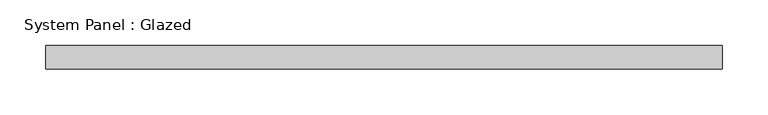
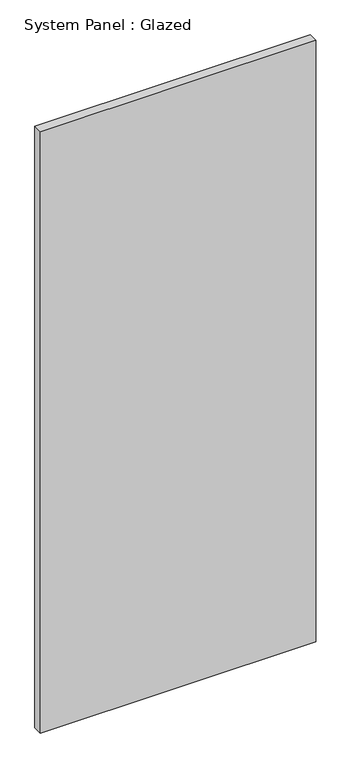
"""IFC4 building model written with IfcOpenShell, lengths in millimetres: plate geometry, System Panel : Glazed."""

from ifc_helpers import new_model, si_unit, origin, origin_with_axes, place, context, project, spatial, polyline, outline, extrude, source, transform, mapped, element, save


def system_panel_glazed_72a11131(model_context):
    return source(origin(), model_context, "Body", "SweptSolid", [
        extrude(outline(polyline([(368.25, 19.05), (-368.25, 19.05), (-368.25, 44.45), (368.25, 44.45), (368.25, 19.05)])), origin_with_axes(), (0.0, 0.0, 1.0), 1701.8),
    ])


if __name__ == "__main__":
    model = new_model("IFC4")
    model_context = context("Model", 3, world=origin())
    ifc_project = project(units=[si_unit("LENGTHUNIT", "METRE", prefix="MILLI")], contexts=[model_context])
    site = spatial("IfcSite", under=ifc_project)
    building = spatial("IfcBuilding", under=site)
    placement = place(None, origin())
    system_panel_glazed_shape = system_panel_glazed_72a11131(model_context)
    element("IfcPlate", 1, ObjectType="System Panel : Glazed", at=placement, inside=building, context=model_context, shape_type="MappedRepresentation", body=[
        mapped(system_panel_glazed_shape, transform((0.0, 0.0, 0.0), x_axis=(1.0, 0.0, 0.0), y_axis=(0.0, 1.0, 0.0), z_axis=(0.0, 0.0, 1.0))),
    ])
    save(model, "model.ifc")

# Revit data of these elements
# Element 1 (IfcPlate, "System Panel : Glazed")
#   Materials on its faces: "Glass"
# Materials
#   "Glass": class "Glass", colour RGB 0 128 192, transparency 0.75
